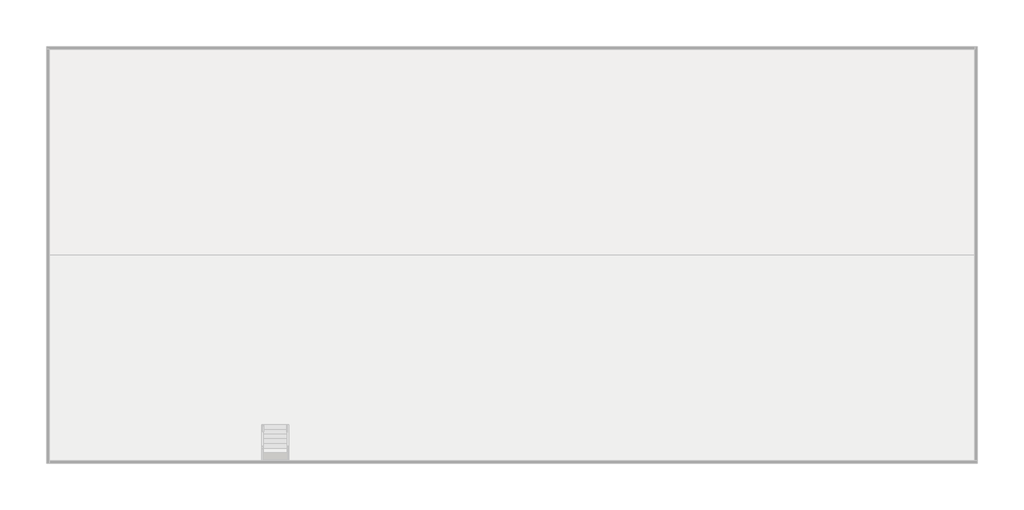
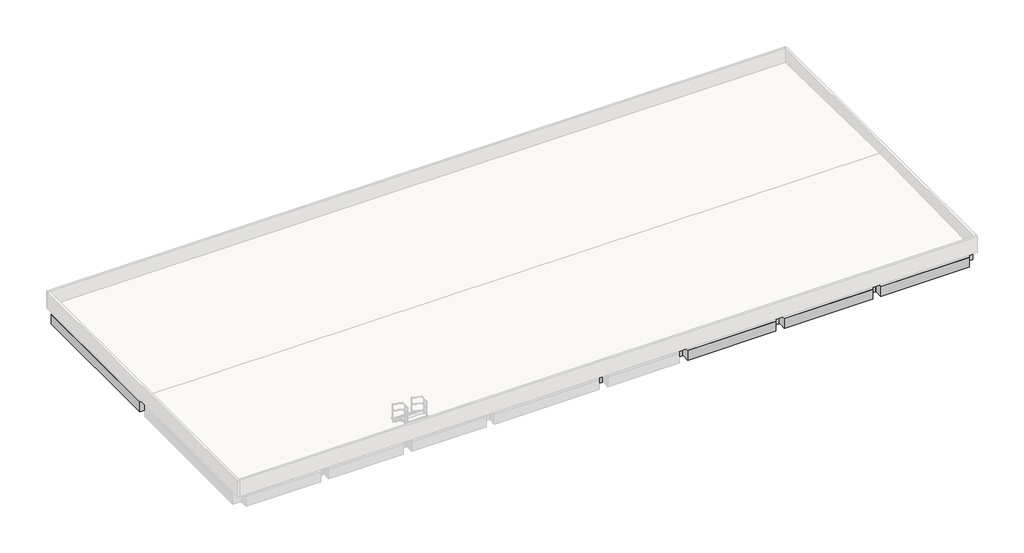
# One storey, part 2 of 3: 33 beams.
"""IFC4 building model written with IfcOpenShell, lengths in millimetres."""

import ifcopenshell
import ifcopenshell.guid

model = None  # the IFC model being written
_history = None  # IfcOwnerHistory: only IFC2X3 demands one
_inside = {}  # id of a spatial element -> (the spatial element, [elements in it])
_under = {}  # id of a project, library or spatial element -> (it, [spatial elements below it])
_declared = {}  # id of a project -> (the project, [libraries it declares])
_typed = {}  # id of a type object -> (the type object, [elements of that type])
_made_of = {}  # id of a material, layer set ... -> (it, [elements and type objects made of it])


def new_model(schema):
    """Start an empty IFC model of exactly this schema.

    Asked for "IFC4X3", IfcOpenShell would pick the latest addendum, in which some entities
    have other attributes; the version numbers below select the first issue.
    IFC2X3 requires an IfcOwnerHistory on every rooted entity: one is made here for all.
    """
    global model, _history
    if schema == "IFC4X3":
        model = ifcopenshell.file(schema_version=(4, 3, 0, 0))
    else:
        model = ifcopenshell.file(schema=schema)
    _inside.clear()
    _under.clear()
    _declared.clear()
    _typed.clear()
    _made_of.clear()
    _history = None
    if model.schema == "IFC2X3":
        org = make("IfcOrganization", Name="unknown")
        user = make(
            "IfcPersonAndOrganization",
            ThePerson=make("IfcPerson", FamilyName="unknown"),
            TheOrganization=org,
        )
        app = make(
            "IfcApplication",
            ApplicationDeveloper=org,
            Version="unknown",
            ApplicationFullName="unknown",
            ApplicationIdentifier="unknown",
        )
        _history = make(
            "IfcOwnerHistory",
            OwningUser=user,
            OwningApplication=app,
            ChangeAction="ADDED",
            CreationDate=0,
        )
    return model


def make(cls, **values):
    """One entity of the class cls with the attributes given. An attribute that is None is left unset."""
    return model.create_entity(
        cls, **{name: value for name, value in values.items() if value is not None}
    )


def rooted(cls, **values):
    """An entity with a GlobalId (a new one), such as an element, a storey or a relation."""
    return make(cls, GlobalId=ifcopenshell.guid.new(), OwnerHistory=_history, **values)


def si_unit(unit_type, name, prefix=None):
    """IfcSIUnit, for example si_unit("LENGTHUNIT", "METRE", prefix="MILLI")."""
    return make("IfcSIUnit", UnitType=unit_type, Prefix=prefix, Name=name)


def assignment(units):
    """IfcUnitAssignment: the units of a project."""
    return None if units is None else make("IfcUnitAssignment", Units=units)


def point(xyz):
    """IfcCartesianPoint."""
    return None if xyz is None else make("IfcCartesianPoint", Coordinates=xyz)


def direction(xyz):
    """IfcDirection."""
    return None if xyz is None else make("IfcDirection", DirectionRatios=xyz)


def frame(location, z_axis=None, x_axis=None):
    """IfcAxis2Placement3D, a coordinate frame: its origin and axes. An axis left out is left unset."""
    return make(
        "IfcAxis2Placement3D",
        Location=point(location),
        Axis=direction(z_axis),
        RefDirection=direction(x_axis),
    )


def origin():
    """The frame at (0, 0, 0) with its axes left unset."""
    return frame((0.0, 0.0, 0.0))


def place(relative_to, where):
    """IfcLocalPlacement: puts the frame where relative to a parent placement (None: the world)."""
    return make(
        "IfcLocalPlacement", PlacementRelTo=relative_to, RelativePlacement=where
    )


def context(
    kind, dimensions, precision=None, world=None, true_north=None, identifier=None
):
    """IfcGeometricRepresentationContext, for example the 3D "Model" context."""
    return make(
        "IfcGeometricRepresentationContext",
        ContextIdentifier=identifier,
        ContextType=kind,
        CoordinateSpaceDimension=dimensions,
        Precision=precision,
        WorldCoordinateSystem=world,
        TrueNorth=true_north,
    )


def project(units=None, contexts=None):
    """IfcProject with its units and contexts."""
    return rooted(
        "IfcProject",
        Name="project",
        RepresentationContexts=contexts,
        UnitsInContext=assignment(units),
    )


def spatial(cls, under=None, at=None, **own):
    """A site, building, storey or space (cls), placed at a placement, below another one or the project."""
    s = rooted(cls, ObjectPlacement=at, **own)
    if under is not None:
        _under.setdefault(under.id(), (under, []))[1].append(s)
    return s


def faces_of(points, faces, orient=None, outer=None):
    """IfcFace entities. A face is a list of loops; a loop is a list of indices into points, from 0.

    orient and outer hold one flag for each loop. By default every Orientation is true, the
    first loop of a face is its IfcFaceOuterBound and the others are IfcFaceBound.
    """
    made = []
    for i, loops in enumerate(faces):
        bounds = []
        for j, loop in enumerate(loops):
            is_outer = j == 0 if outer is None else outer[i][j]
            bounds.append(
                make(
                    "IfcFaceOuterBound" if is_outer else "IfcFaceBound",
                    Bound=make("IfcPolyLoop", Polygon=[points[k] for k in loop]),
                    Orientation=True if orient is None else orient[i][j],
                )
            )
        made.append(make("IfcFace", Bounds=bounds))
    return made


def faceted_brep(points, faces, orient=None, outer=None, voids=None):
    """IfcFacetedBrep: a solid bounded by flat faces; with voids (closed shells), ...WithVoids."""
    shared = [point(p) for p in points]
    hull = make("IfcClosedShell", CfsFaces=faces_of(shared, faces, orient, outer))
    if voids is None:
        return make("IfcFacetedBrep", Outer=hull)
    return make(
        "IfcFacetedBrepWithVoids",
        Outer=hull,
        Voids=[
            make(cls, CfsFaces=faces_of(shared, fs, o, b)) for cls, fs, o, b in voids
        ],
    )


def shape(context_of_items, identifier, shape_type, items):
    """IfcShapeRepresentation: the items that make up one representation, for example the "Body"."""
    return make(
        "IfcShapeRepresentation",
        ContextOfItems=context_of_items,
        RepresentationIdentifier=identifier,
        RepresentationType=shape_type,
        Items=items,
    )


def made_of(thing, what):
    """Note that an element or type object is made of a material, layer set ...; save() writes the relation."""
    if what is not None:
        _made_of.setdefault(what.id(), (what, []))[1].append(thing)
    return thing


def element(
    cls,
    number,
    at=None,
    inside=None,
    cuts=None,
    type_object=None,
    material=None,
    context=None,
    identifier="Body",
    shape_type=None,
    held_by="IfcProductDefinitionShape",
    body=None,
    shapes=None,
    **own,
):
    """One element of the class cls, such as IfcWall. Its Tag is "e" and its number.

    at: its placement. inside: the storey or other place that contains it. cuts: it is an
    opening in that element (IfcRelVoidsElement). A single representation is given by context,
    identifier, shape_type and body (its items); several are given by shapes. held_by: the class
    of the entity that holds the representations. save() writes the other relations.
    """
    e = rooted(cls, Tag="e%d" % number, ObjectPlacement=at, **own)
    if body is not None:
        shapes = [shape(context, identifier, shape_type, body)]
    if shapes is not None:
        e.Representation = make(held_by, Representations=shapes)
    if inside is not None:
        _inside.setdefault(inside.id(), (inside, []))[1].append(e)
    if cuts is not None:
        rooted(
            "IfcRelVoidsElement", RelatingBuildingElement=cuts, RelatedOpeningElement=e
        )
    if type_object is not None:
        _typed.setdefault(type_object.id(), (type_object, []))[1].append(e)
    return made_of(e, material)


def aggregate(whole, parts):
    """IfcRelAggregates: a whole, such as a stair, and the parts it consists of."""
    return rooted("IfcRelAggregates", RelatingObject=whole, RelatedObjects=parts)


def save(model, path):
    """Write the relations noted so far, then the file.

    IfcRelAggregates (storeys below a building ...), IfcRelContainedInSpatialStructure (elements
    in a storey), IfcRelDefinesByType, IfcRelAssociatesMaterial and IfcRelDeclares: one each for
    every whole, place, type object, material and project.
    """
    for whole, parts in _under.values():
        aggregate(whole, parts)
    for where, things in _inside.values():
        rooted(
            "IfcRelContainedInSpatialStructure",
            RelatedElements=things,
            RelatingStructure=where,
        )
    for kind, things in _typed.values():
        rooted("IfcRelDefinesByType", RelatedObjects=things, RelatingType=kind)
    for what, things in _made_of.values():
        rooted("IfcRelAssociatesMaterial", RelatedObjects=things, RelatingMaterial=what)
    for by, libraries in _declared.values():
        rooted("IfcRelDeclares", RelatingContext=by, RelatedDefinitions=libraries)
    model.write(path)


model = new_model("IFC4")

# Units and contexts
model_context = context("Model", 3, world=origin())
ifc_project = project(units=[si_unit("LENGTHUNIT", "METRE", prefix="MILLI")], contexts=[model_context])

# Site, building, storey
site = spatial("IfcSite", under=ifc_project)
building = spatial("IfcBuilding", under=site)
storey = spatial("IfcBuildingStorey", under=building, Name="TOC", Elevation=7649.9618634)

# Beams
placement = place(None, origin())
element("IfcBeam", 1, ObjectType="RC Beam_Rectangular : H_SB_AR_S16_B600xH900_RG9", at=placement, inside=storey, context=model_context, shape_type="Brep", body=[
    faceted_brep([(300.0, 24199.5208589, 6749.9618634), (300.0, 23749.5208589, 6749.9618634), (300.0, 23599.5208589, 6749.9618634), (300.0, 23599.5208589, 7499.9618634), (300.0, 24199.5208589, 7499.9618634), (5700.0, 23599.5208589, 6749.9618634), (5700.0, 23749.5208589, 6749.9618634), (5700.0, 24199.5208589, 6749.9618634), (5700.0, 24199.5208589, 7499.9618634), (5700.0, 23599.5208589, 7499.9618634), (2800.0, 23599.5208589, 7499.9618634), (3200.0, 23599.5208589, 7499.9618634), (2800.0, 23599.5208589, 6749.9618634), (3200.0, 23599.5208589, 6749.9618634)], [[[0, 1, 2, 3, 4]], [[5, 6, 7, 8, 9]], [[4, 3, 10, 11, 9, 8]], [[2, 12, 13, 5, 9, 11, 10, 3]], [[2, 1, 0, 7, 6, 5, 13, 12]], [[7, 0, 4, 8]]]),
])
element("IfcBeam", 2, ObjectType="RC Beam_Rectangular : H_SB_AR_S16_B600xH900_RG9", at=placement, inside=storey, context=model_context, shape_type="Brep", body=[
    faceted_brep([(6300.0, 24199.5208589, 6749.9618634), (6300.0, 23749.5208589, 6749.9618634), (6300.0, 23599.5208589, 6749.9618634), (6300.0, 23599.5208589, 7499.9618634), (6300.0, 24199.5208589, 7499.9618634), (11700.0, 23599.5208589, 6749.9618634), (11700.0, 23749.5208589, 6749.9618634), (11700.0, 24199.5208589, 6749.9618634), (11700.0, 24199.5208589, 7499.9618634), (11700.0, 23599.5208589, 7499.9618634), (8800.0, 23599.5208589, 7499.9618634), (9200.0, 23599.5208589, 7499.9618634), (8800.0, 23599.5208589, 6749.9618634), (9200.0, 23599.5208589, 6749.9618634)], [[[0, 1, 2, 3, 4]], [[5, 6, 7, 8, 9]], [[4, 3, 10, 11, 9, 8]], [[2, 12, 13, 5, 9, 11, 10, 3]], [[2, 1, 0, 7, 6, 5, 13, 12]], [[7, 0, 4, 8]]]),
])
element("IfcBeam", 3, ObjectType="RC Beam_Rectangular : H_SB_AR_S16_B600xH900_RG9", at=placement, inside=storey, context=model_context, shape_type="Brep", body=[
    faceted_brep([(12300.0, 24199.5208589, 6749.9618634), (12300.0, 23749.5208589, 6749.9618634), (12300.0, 23599.5208589, 6749.9618634), (12300.0, 23599.5208589, 7499.9618634), (12300.0, 24199.5208589, 7499.9618634), (17700.0, 23599.5208589, 6749.9618634), (17700.0, 23749.5208589, 6749.9618634), (17700.0, 24199.5208589, 6749.9618634), (17700.0, 24199.5208589, 7499.9618634), (17700.0, 23599.5208589, 7499.9618634), (14800.0, 23599.5208589, 7499.9618634), (15200.0, 23599.5208589, 7499.9618634), (14800.0, 23599.5208589, 6749.9618634), (15200.0, 23599.5208589, 6749.9618634)], [[[0, 1, 2, 3, 4]], [[5, 6, 7, 8, 9]], [[4, 3, 10, 11, 9, 8]], [[2, 12, 13, 5, 9, 11, 10, 3]], [[2, 1, 0, 7, 6, 5, 13, 12]], [[7, 0, 4, 8]]]),
])
element("IfcBeam", 4, ObjectType="RC Beam_Rectangular : H_SB_AR_S16_B600xH900_RG9", at=placement, inside=storey, context=model_context, shape_type="Brep", body=[
    faceted_brep([(18300.0, 24199.5208589, 6749.9618634), (18300.0, 23749.5208589, 6749.9618634), (18300.0, 23599.5208589, 6749.9618634), (18300.0, 23599.5208589, 7499.9618634), (18300.0, 24199.5208589, 7499.9618634), (25900.0, 23599.5208589, 6749.9618634), (25900.0, 23749.5208589, 6749.9618634), (25900.0, 24199.5208589, 6749.9618634), (25900.0, 24199.5208589, 7499.9618634), (25900.0, 23599.5208589, 7499.9618634), (21800.0, 23599.5208589, 7499.9618634), (22400.0, 23599.5208589, 7499.9618634), (21800.0, 23599.5208589, 6749.9618634), (22400.0, 23599.5208589, 6749.9618634)], [[[0, 1, 2, 3, 4]], [[5, 6, 7, 8, 9]], [[4, 3, 10, 11, 9, 8]], [[2, 12, 13, 5, 9, 11, 10, 3]], [[2, 1, 0, 7, 6, 5, 13, 12]], [[7, 0, 4, 8]]]),
])
element("IfcBeam", 5, ObjectType="RC Beam_Rectangular : H_SB_AR_S16_B600xH900_RG9", at=placement, inside=storey, context=model_context, shape_type="Brep", body=[
    faceted_brep([(26500.0, 24199.5208589, 6749.9618634), (26500.0, 23749.5208589, 6749.9618634), (26500.0, 23599.5208589, 6749.9618634), (26500.0, 23599.5208589, 7499.9618634), (26500.0, 24199.5208589, 7499.9618634), (31700.0, 23599.5208589, 6749.9618634), (31700.0, 23749.5208589, 6749.9618634), (31700.0, 24199.5208589, 6749.9618634), (31700.0, 24199.5208589, 7499.9618634), (31700.0, 23599.5208589, 7499.9618634), (28800.0, 23599.5208589, 7499.9618634), (29400.0, 23599.5208589, 7499.9618634), (28800.0, 23599.5208589, 6749.9618634), (29400.0, 23599.5208589, 6749.9618634)], [[[0, 1, 2, 3, 4]], [[5, 6, 7, 8, 9]], [[4, 3, 10, 11, 9, 8]], [[2, 12, 13, 5, 9, 11, 10, 3]], [[2, 1, 0, 7, 6, 5, 13, 12]], [[7, 0, 4, 8]]]),
])
element("IfcBeam", 6, ObjectType="RC Beam_Rectangular : H_SB_AR_S16_B600xH900_RG5", at=placement, inside=storey, context=model_context, shape_type="Brep", body=[
    faceted_brep([(26500.0, 8599.5208589, 6749.9618634), (26500.0, 8399.5208589, 6749.9618634), (26500.0, 7999.5208589, 6749.9618634), (26500.0, 7999.5208589, 7499.9618634), (26500.0, 8599.5208589, 7499.9618634), (31700.0, 7999.5208589, 6749.9618634), (31700.0, 8399.5208589, 6749.9618634), (31700.0, 8599.5208589, 6749.9618634), (31700.0, 8599.5208589, 7499.9618634), (31700.0, 7999.5208589, 7499.9618634), (28500.0, 7999.5208589, 7499.9618634), (28700.0, 7999.5208589, 7499.9618634), (28800.0, 7999.5208589, 7499.9618634), (29400.0, 7999.5208589, 7499.9618634), (29400.0, 8599.5208589, 7499.9618634), (28800.0, 8599.5208589, 7499.9618634), (28500.0, 7999.5208589, 6749.9618634), (28700.0, 7999.5208589, 6749.9618634), (28800.0, 7999.5208589, 6749.9618634), (29400.0, 7999.5208589, 6749.9618634), (28800.0, 8599.5208589, 6749.9618634), (29400.0, 8599.5208589, 6749.9618634)], [[[0, 1, 2, 3, 4]], [[5, 6, 7, 8, 9]], [[4, 3, 10, 11, 12, 13, 9, 8, 14, 15]], [[2, 16, 17, 18, 19, 5, 9, 13, 12, 11, 10, 3]], [[2, 1, 0, 20, 21, 7, 6, 5, 19, 18, 17, 16]], [[7, 21, 20, 0, 4, 15, 14, 8]]]),
])
element("IfcBeam", 7, ObjectType="RC Beam_Rectangular : H_SB_AR_S16_B600xH900_RG5", at=placement, inside=storey, context=model_context, shape_type="Brep", body=[
    faceted_brep([(32300.0, 8599.5208589, 6749.9618634), (32300.0, 8399.5208589, 6749.9618634), (32300.0, 7999.5208589, 6749.9618634), (32300.0, 7999.5208589, 7499.9618634), (32300.0, 8599.5208589, 7499.9618634), (38700.0, 7999.5208589, 6749.9618634), (38700.0, 8599.5208589, 6749.9618634), (38700.0, 8599.5208589, 7499.9618634), (38700.0, 7999.5208589, 7499.9618634), (35200.0, 7999.5208589, 7499.9618634), (35800.0, 7999.5208589, 7499.9618634), (36500.0, 7999.5208589, 7499.9618634), (36700.0, 7999.5208589, 7499.9618634), (36700.0, 8599.5208589, 7499.9618634), (36500.0, 8599.5208589, 7499.9618634), (35800.0, 8599.5208589, 7499.9618634), (35200.0, 8599.5208589, 7499.9618634), (33450.0, 8599.5208589, 7499.9618634), (33250.0, 8599.5208589, 7499.9618634), (35200.0, 7999.5208589, 6749.9618634), (35800.0, 7999.5208589, 6749.9618634), (36500.0, 7999.5208589, 6749.9618634), (36700.0, 7999.5208589, 6749.9618634), (35200.0, 8599.5208589, 6749.9618634), (35800.0, 8599.5208589, 6749.9618634), (36500.0, 8599.5208589, 6749.9618634), (36700.0, 8599.5208589, 6749.9618634)], [[[0, 1, 2, 3, 4]], [[5, 6, 7, 8]], [[4, 3, 9, 10, 11, 12, 8, 7, 13, 14, 15, 16, 17, 18]], [[2, 19, 20, 21, 22, 5, 8, 12, 11, 10, 9, 3]], [[2, 1, 0, 23, 24, 25, 26, 6, 5, 22, 21, 20, 19]], [[6, 26, 25, 24, 23, 0, 4, 18, 17, 16, 15, 14, 13, 7]]]),
])
element("IfcBeam", 8, ObjectType="RC Beam_Rectangular : H_SB_AR_S16_B600xH900_RG5", at=placement, inside=storey, context=model_context, shape_type="Brep", body=[
    faceted_brep([(39300.0, 8599.5208589, 6749.9618634), (39300.0, 8404.5208589, 6749.9618634), (39300.0, 8204.5208589, 6749.9618634), (39300.0, 7999.5208589, 6749.9618634), (39300.0, 7999.5208589, 7499.9618634), (39300.0, 8599.5208589, 7499.9618634), (45700.0, 7999.5208589, 6749.9618634), (45700.0, 8399.5208589, 6749.9618634), (45700.0, 8599.5208589, 6749.9618634), (45700.0, 8599.5208589, 7499.9618634), (45700.0, 7999.5208589, 7499.9618634), (41925.0, 7999.5208589, 7499.9618634), (42125.0, 7999.5208589, 7499.9618634), (42200.0, 7999.5208589, 7499.9618634), (42800.0, 7999.5208589, 7499.9618634), (43200.0, 7999.5208589, 7499.9618634), (43400.0, 7999.5208589, 7499.9618634), (42800.0, 8599.5208589, 7499.9618634), (42200.0, 8599.5208589, 7499.9618634), (41925.0, 7999.5208589, 6749.9618634), (42125.0, 7999.5208589, 6749.9618634), (42200.0, 7999.5208589, 6749.9618634), (42800.0, 7999.5208589, 6749.9618634), (43200.0, 7999.5208589, 6749.9618634), (43400.0, 7999.5208589, 6749.9618634), (42200.0, 8599.5208589, 6749.9618634), (42800.0, 8599.5208589, 6749.9618634), (45640.0, 8599.5208589, 6749.9618634)], [[[0, 1, 2, 3, 4, 5]], [[6, 7, 8, 9, 10]], [[5, 4, 11, 12, 13, 14, 15, 16, 10, 9, 17, 18]], [[3, 19, 20, 21, 22, 23, 24, 6, 10, 16, 15, 14, 13, 12, 11, 4]], [[3, 2, 1, 0, 25, 26, 27, 8, 7, 6, 24, 23, 22, 21, 20, 19]], [[8, 27, 26, 25, 0, 5, 18, 17, 9]]]),
])
element("IfcBeam", 9, ObjectType="RC Beam_Rectangular : H_SB_AR_S16_B600xH900_RG5", at=placement, inside=storey, context=model_context, shape_type="Brep", body=[
    faceted_brep([(46300.0, 8599.5208589, 6749.9618634), (46300.0, 8399.5208589, 6749.9618634), (46300.0, 7999.5208589, 6749.9618634), (46300.0, 7999.5208589, 7499.9618634), (46300.0, 8599.5208589, 7499.9618634), (52700.0, 7999.5208589, 6749.9618634), (52700.0, 8399.5208589, 6749.9618634), (52700.0, 8599.5208589, 6749.9618634), (52700.0, 8599.5208589, 7499.9618634), (52700.0, 7999.5208589, 7499.9618634), (49200.0, 7999.5208589, 7499.9618634), (49800.0, 7999.5208589, 7499.9618634), (52574.0, 7999.5208589, 7499.9618634), (52574.0, 8599.5208589, 7499.9618634), (50725.0, 8599.5208589, 7499.9618634), (50525.0, 8599.5208589, 7499.9618634), (49800.0, 8599.5208589, 7499.9618634), (49200.0, 8599.5208589, 7499.9618634), (49200.0, 7999.5208589, 6749.9618634), (49800.0, 7999.5208589, 6749.9618634), (52574.0, 7999.5208589, 6749.9618634), (49200.0, 8599.5208589, 6749.9618634), (49800.0, 8599.5208589, 6749.9618634)], [[[0, 1, 2, 3, 4]], [[5, 6, 7, 8, 9]], [[4, 3, 10, 11, 12, 9, 8, 13, 14, 15, 16, 17]], [[2, 18, 19, 20, 5, 9, 12, 11, 10, 3]], [[2, 1, 0, 21, 22, 7, 6, 5, 20, 19, 18]], [[7, 22, 21, 0, 4, 17, 16, 15, 14, 13, 8]]]),
])
element("IfcBeam", 10, ObjectType="RC Beam_Rectangular : H_SB_AR_S16_B600xH900_RG9", at=placement, inside=storey, context=model_context, shape_type="Brep", body=[
    faceted_brep([(32300.0, 799.5208589, 6749.9618634), (32300.0, 649.5208589, 6749.9618634), (32300.0, 199.5208589, 6749.9618634), (32300.0, 199.5208589, 7499.9618634), (32300.0, 799.5208589, 7499.9618634), (38700.0, 199.5208589, 6749.9618634), (38700.0, 649.5208589, 6749.9618634), (38700.0, 799.5208589, 6749.9618634), (38700.0, 799.5208589, 7499.9618634), (38700.0, 199.5208589, 7499.9618634), (36700.0, 799.5208589, 7499.9618634), (36500.0, 799.5208589, 7499.9618634), (35800.0, 799.5208589, 7499.9618634), (35200.0, 799.5208589, 7499.9618634), (35200.0, 799.5208589, 6749.9618634), (35800.0, 799.5208589, 6749.9618634)], [[[0, 1, 2, 3, 4]], [[5, 6, 7, 8, 9]], [[4, 3, 9, 8, 10, 11, 12, 13]], [[2, 5, 9, 3]], [[2, 1, 0, 14, 15, 7, 6, 5]], [[7, 15, 14, 0, 4, 13, 12, 11, 10, 8]]]),
])
element("IfcBeam", 11, ObjectType="RC Beam_Rectangular : H_SB_AR_S16_B600xH900_RG9", at=placement, inside=storey, context=model_context, shape_type="Brep", body=[
    faceted_brep([(39300.0, 799.5208589, 6749.9618634), (39300.0, 649.5208589, 6749.9618634), (39300.0, 199.5208589, 6749.9618634), (39300.0, 199.5208589, 7499.9618634), (39300.0, 799.5208589, 7499.9618634), (45700.0, 199.5208589, 6749.9618634), (45700.0, 649.5208589, 6749.9618634), (45700.0, 799.5208589, 6749.9618634), (45700.0, 799.5208589, 7499.9618634), (45700.0, 199.5208589, 7499.9618634), (43400.0, 799.5208589, 7499.9618634), (43200.0, 799.5208589, 7499.9618634), (42800.0, 799.5208589, 7499.9618634), (42200.0, 799.5208589, 7499.9618634), (42200.0, 799.5208589, 6749.9618634), (42800.0, 799.5208589, 6749.9618634)], [[[0, 1, 2, 3, 4]], [[5, 6, 7, 8, 9]], [[4, 3, 9, 8, 10, 11, 12, 13]], [[2, 5, 9, 3]], [[2, 1, 0, 14, 15, 7, 6, 5]], [[7, 15, 14, 0, 4, 13, 12, 11, 10, 8]]]),
])
element("IfcBeam", 12, ObjectType="RC Beam_Rectangular : H_SB_AR_S16_B600xH900_RG9", at=placement, inside=storey, context=model_context, shape_type="Brep", body=[
    faceted_brep([(46300.0, 799.5208589, 6749.9618634), (46300.0, 649.5208589, 6749.9618634), (46300.0, 199.5208589, 6749.9618634), (46300.0, 199.5208589, 7499.9618634), (46300.0, 799.5208589, 7499.9618634), (52700.0, 199.5208589, 6749.9618634), (52700.0, 649.5208589, 6749.9618634), (52700.0, 799.5208589, 6749.9618634), (52700.0, 799.5208589, 7499.9618634), (52700.0, 199.5208589, 7499.9618634), (49800.0, 799.5208589, 7499.9618634), (49200.0, 799.5208589, 7499.9618634), (46800.0, 799.5208589, 7499.9618634), (46600.0, 799.5208589, 7499.9618634), (49200.0, 799.5208589, 6749.9618634), (49800.0, 799.5208589, 6749.9618634)], [[[0, 1, 2, 3, 4]], [[5, 6, 7, 8, 9]], [[4, 3, 9, 8, 10, 11, 12, 13]], [[2, 5, 9, 3]], [[2, 1, 0, 14, 15, 7, 6, 5]], [[7, 15, 14, 0, 4, 13, 12, 11, 10, 8]]]),
])
element("IfcBeam", 13, ObjectType="RC Beam_Rectangular : H_SB_AR_S16_B600xH900_RG6", at=placement, inside=storey, context=model_context, shape_type="Brep", body=[
    faceted_brep([(-300.0, 12499.5208589, 6749.9618634), (150.0, 12499.5208589, 6749.9618634), (300.0, 12499.5208589, 6749.9618634), (300.0, 12499.5208589, 7499.9618634), (-300.0, 12499.5208589, 7499.9618634), (300.0, 23599.5208589, 6749.9618634), (150.0, 23599.5208589, 6749.9618634), (-300.0, 23599.5208589, 6749.9618634), (-300.0, 23599.5208589, 7499.9618634), (300.0, 23599.5208589, 7499.9618634), (300.0, 23473.5208589, 7499.9618634)], [[[0, 1, 2, 3, 4]], [[5, 6, 7, 8, 9]], [[4, 3, 10, 9, 8]], [[2, 5, 9, 10, 3]], [[2, 1, 0, 7, 6, 5]], [[7, 0, 4, 8]]]),
])
element("IfcBeam", 14, ObjectType="RC Beam_Rectangular : H_SB_AR_S16_B400xH900_RG1", at=placement, inside=storey, context=model_context, shape_type="Brep", body=[
    faceted_brep([(6200.0, 23599.5208589, 7499.9618634), (5800.0, 23599.5208589, 7499.9618634), (5800.0, 23473.5208589, 7499.9618634), (5800.0, 12499.5208589, 7499.9618634), (6200.0, 12499.5208589, 7499.9618634), (6200.0, 23473.5208589, 7499.9618634), (6200.0, 23599.5208589, 6749.9618634), (5800.0, 23599.5208589, 6749.9618634), (5800.0, 12499.5208589, 6749.9618634), (6200.0, 12499.5208589, 6749.9618634), (6200.0, 23473.5208589, 6749.9618634), (5800.0, 23473.5208589, 6749.9618634)], [[[0, 1, 2, 3, 4, 5]], [[6, 7, 1, 0]], [[8, 9, 4, 3]], [[9, 10, 6, 0, 5, 4]], [[8, 11, 7, 6, 10, 9]], [[7, 11, 8, 3, 2, 1]]]),
])
element("IfcBeam", 15, ObjectType="RC Beam_Rectangular : H_SB_AR_S16_B400xH900_RG1", at=placement, inside=storey, context=model_context, shape_type="Brep", body=[
    faceted_brep([(12200.0, 23599.5208589, 7499.9618634), (11800.0, 23599.5208589, 7499.9618634), (11800.0, 23473.5208589, 7499.9618634), (11800.0, 12499.5208589, 7499.9618634), (12200.0, 12499.5208589, 7499.9618634), (12200.0, 23473.5208589, 7499.9618634), (12200.0, 23599.5208589, 6749.9618634), (11800.0, 23599.5208589, 6749.9618634), (11800.0, 12499.5208589, 6749.9618634), (12200.0, 12499.5208589, 6749.9618634), (12200.0, 23473.5208589, 6749.9618634), (11800.0, 23473.5208589, 6749.9618634)], [[[0, 1, 2, 3, 4, 5]], [[6, 7, 1, 0]], [[8, 9, 4, 3]], [[9, 10, 6, 0, 5, 4]], [[9, 8, 11, 7, 6, 10]], [[7, 11, 8, 3, 2, 1]]]),
])
element("IfcBeam", 16, ObjectType="RC Beam_Rectangular : H_SB_AR_S16_B600xH900_RG1A", at=placement, inside=storey, context=model_context, shape_type="Brep", body=[
    faceted_brep([(17700.0, 12499.5208589, 6749.9618634), (18100.0, 12499.5208589, 6749.9618634), (18300.0, 12499.5208589, 6749.9618634), (18300.0, 12499.5208589, 7499.9618634), (17700.0, 12499.5208589, 7499.9618634), (18300.0, 23473.5208589, 7499.9618634), (18300.0, 23599.5208589, 7499.9618634), (17700.0, 23599.5208589, 7499.9618634), (17700.0, 23473.5208589, 7499.9618634), (18300.0, 23599.5208589, 6749.9618634), (18100.0, 23599.5208589, 6749.9618634), (17700.0, 23599.5208589, 6749.9618634), (17700.0, 23473.5208589, 6749.9618634)], [[[0, 1, 2, 3, 4]], [[4, 3, 5, 6, 7, 8]], [[9, 10, 11, 7, 6]], [[2, 9, 6, 5, 3]], [[0, 12, 11, 10, 9, 2, 1]], [[11, 12, 0, 4, 8, 7]]]),
])
element("IfcBeam", 17, ObjectType="RC Beam_Rectangular : H_SB_AR_S16_B500xH900_RG3", at=placement, inside=storey, context=model_context, shape_type="Brep", body=[
    faceted_brep([(26450.0, 7999.5208589, 6749.9618634), (26300.0, 7999.5208589, 6749.9618634), (26100.0, 7999.5208589, 6749.9618634), (25950.0, 7999.5208589, 6749.9618634), (25950.0, 7999.5208589, 7499.9618634), (26450.0, 7999.5208589, 7499.9618634), (25950.0, 925.5208589, 7499.9618634), (25950.0, 799.5208589, 7499.9618634), (26450.0, 799.5208589, 7499.9618634), (26450.0, 925.5208589, 7499.9618634), (26450.0, 2637.0208589, 7499.9618634), (26450.0, 2837.0208589, 7499.9618634), (25950.0, 799.5208589, 6749.9618634), (26100.0, 799.5208589, 6749.9618634), (26300.0, 799.5208589, 6749.9618634), (26450.0, 799.5208589, 6749.9618634), (26450.0, 925.5208589, 6749.9618634), (26450.0, 2637.0208589, 6749.9618634), (26450.0, 2837.0208589, 6749.9618634), (25950.0, 925.5208589, 6749.9618634)], [[[0, 1, 2, 3, 4, 5]], [[5, 4, 6, 7, 8, 9, 10, 11]], [[12, 13, 14, 15, 8, 7]], [[15, 16, 17, 18, 0, 5, 11, 10, 9, 8]], [[12, 19, 3, 2, 1, 0, 18, 17, 16, 15, 14, 13]], [[3, 19, 12, 7, 6, 4]]]),
])
element("IfcBeam", 18, ObjectType="RC Beam_Rectangular : H_SB_AR_S16_B500xH900_RG2", at=placement, inside=storey, context=model_context, shape_type="Brep", body=[
    faceted_brep([(26450.0, 23599.5208589, 7499.9618634), (25950.0, 23599.5208589, 7499.9618634), (25950.0, 23473.5208589, 7499.9618634), (25950.0, 8599.5208589, 7499.9618634), (26450.0, 8599.5208589, 7499.9618634), (26450.0, 23473.5208589, 7499.9618634), (26450.0, 23599.5208589, 6749.9618634), (25950.0, 23599.5208589, 6749.9618634), (25950.0, 8599.5208589, 6749.9618634), (26450.0, 8599.5208589, 6749.9618634), (26450.0, 23473.5208589, 6749.9618634), (25950.0, 23473.5208589, 6749.9618634)], [[[0, 1, 2, 3, 4, 5]], [[6, 7, 1, 0]], [[8, 9, 4, 3]], [[9, 10, 6, 0, 5, 4]], [[6, 10, 9, 8, 11, 7]], [[7, 11, 8, 3, 2, 1]]]),
])
element("IfcBeam", 19, ObjectType="RC Beam_Rectangular : H_SB_AR_S16_B500xH900_RG3", at=placement, inside=storey, context=model_context, shape_type="Brep", body=[
    faceted_brep([(31750.0, 799.5208589, 7499.9618634), (32250.0, 799.5208589, 7499.9618634), (32250.0, 925.5208589, 7499.9618634), (32250.0, 7999.5208589, 7499.9618634), (31750.0, 7999.5208589, 7499.9618634), (31750.0, 799.5208589, 6749.9618634), (31900.0, 799.5208589, 6749.9618634), (32250.0, 799.5208589, 6749.9618634), (32250.0, 7999.5208589, 6749.9618634), (31900.0, 7999.5208589, 6749.9618634), (31750.0, 7999.5208589, 6749.9618634), (32250.0, 925.5208589, 6749.9618634)], [[[0, 1, 2, 3, 4]], [[5, 6, 7, 1, 0]], [[8, 9, 10, 4, 3]], [[7, 11, 8, 3, 2, 1]], [[5, 10, 9, 8, 11, 7, 6]], [[10, 5, 0, 4]]]),
])
element("IfcBeam", 20, ObjectType="RC Beam_Rectangular : H_SB_AR_S16_B500xH900_RG2", at=placement, inside=storey, context=model_context, shape_type="Brep", body=[
    faceted_brep([(32250.0, 23599.5208589, 7499.9618634), (31750.0, 23599.5208589, 7499.9618634), (31750.0, 23473.5208589, 7499.9618634), (31750.0, 8599.5208589, 7499.9618634), (32250.0, 8599.5208589, 7499.9618634), (32250.0, 23473.5208589, 7499.9618634), (32250.0, 23599.5208589, 6749.9618634), (31750.0, 23599.5208589, 6749.9618634), (31750.0, 8599.5208589, 6749.9618634), (32250.0, 8599.5208589, 6749.9618634), (32250.0, 23473.5208589, 6749.9618634), (31750.0, 23473.5208589, 6749.9618634)], [[[0, 1, 2, 3, 4, 5]], [[6, 7, 1, 0]], [[8, 9, 4, 3]], [[9, 10, 6, 0, 5, 4]], [[8, 11, 7, 6, 10, 9]], [[7, 11, 8, 3, 2, 1]]]),
])
element("IfcBeam", 21, ObjectType="RC Beam_Rectangular : H_SB_AR_S16_B500xH900_RG3", at=placement, inside=storey, context=model_context, shape_type="Brep", body=[
    faceted_brep([(38750.0, 799.5208589, 7499.9618634), (39250.0, 799.5208589, 7499.9618634), (39250.0, 925.5208589, 7499.9618634), (39250.0, 4649.5208589, 7499.9618634), (39250.0, 4849.5208589, 7499.9618634), (39250.0, 7999.5208589, 7499.9618634), (38750.0, 7999.5208589, 7499.9618634), (38750.0, 3543.8249516, 7499.9618634), (38750.0, 3343.8249516, 7499.9618634), (38750.0, 925.5208589, 7499.9618634), (38750.0, 799.5208589, 6749.9618634), (38900.0, 799.5208589, 6749.9618634), (39100.0, 799.5208589, 6749.9618634), (39250.0, 799.5208589, 6749.9618634), (39250.0, 7999.5208589, 6749.9618634), (39100.0, 7999.5208589, 6749.9618634), (38900.0, 7999.5208589, 6749.9618634), (38750.0, 7999.5208589, 6749.9618634), (39250.0, 925.5208589, 6749.9618634), (39250.0, 4649.5208589, 6749.9618634), (39250.0, 4849.5208589, 6749.9618634), (38750.0, 925.5208589, 6749.9618634), (38750.0, 3343.8249516, 6749.9618634), (38750.0, 3543.8249516, 6749.9618634)], [[[0, 1, 2, 3, 4, 5, 6, 7, 8, 9]], [[10, 11, 12, 13, 1, 0]], [[14, 15, 16, 17, 6, 5]], [[13, 18, 19, 20, 14, 5, 4, 3, 2, 1]], [[10, 21, 22, 23, 17, 16, 15, 14, 20, 19, 18, 13, 12, 11]], [[17, 23, 22, 21, 10, 0, 9, 8, 7, 6]]]),
])
element("IfcBeam", 22, ObjectType="RC Beam_Rectangular : H_SB_AR_S16_B500xH900_RG3", at=placement, inside=storey, context=model_context, shape_type="Brep", body=[
    faceted_brep([(45750.0, 799.5208589, 7499.9618634), (46250.0, 799.5208589, 7499.9618634), (46250.0, 925.5208589, 7499.9618634), (46250.0, 4649.5208589, 7499.9618634), (46250.0, 4849.5208589, 7499.9618634), (46250.0, 6599.5208589, 7499.9618634), (46250.0, 6799.5208589, 7499.9618634), (46250.0, 7999.5208589, 7499.9618634), (45750.0, 7999.5208589, 7499.9618634), (45750.0, 6799.5208589, 7499.9618634), (45750.0, 6599.5208589, 7499.9618634), (45750.0, 4849.5208589, 7499.9618634), (45750.0, 4649.5208589, 7499.9618634), (45750.0, 925.5208589, 7499.9618634), (45750.0, 799.5208589, 6749.9618634), (46250.0, 799.5208589, 6749.9618634), (46250.0, 7999.5208589, 6749.9618634), (45750.0, 7999.5208589, 6749.9618634), (46250.0, 925.5208589, 6749.9618634), (46250.0, 4649.5208589, 6749.9618634), (46250.0, 4849.5208589, 6749.9618634), (46250.0, 6599.5208589, 6749.9618634), (46250.0, 6799.5208589, 6749.9618634), (45750.0, 925.5208589, 6749.9618634), (45750.0, 4649.5208589, 6749.9618634), (45750.0, 4849.5208589, 6749.9618634), (45750.0, 6599.5208589, 6749.9618634), (45750.0, 6799.5208589, 6749.9618634)], [[[0, 1, 2, 3, 4, 5, 6, 7, 8, 9, 10, 11, 12, 13]], [[14, 15, 1, 0]], [[16, 17, 8, 7]], [[15, 18, 19, 20, 21, 22, 16, 7, 6, 5, 4, 3, 2, 1]], [[14, 23, 24, 25, 26, 27, 17, 16, 22, 21, 20, 19, 18, 15]], [[17, 27, 26, 25, 24, 23, 14, 0, 13, 12, 11, 10, 9, 8]]]),
])
element("IfcBeam", 23, ObjectType="RC Beam_Rectangular : H_SB_AR_S16_B600xH900_RG8", at=placement, inside=storey, context=model_context, shape_type="Brep", body=[
    faceted_brep([(53300.0, 7999.5208589, 6749.9618634), (52850.0, 7999.5208589, 6749.9618634), (52700.0, 7999.5208589, 6749.9618634), (52700.0, 7999.5208589, 7499.9618634), (53300.0, 7999.5208589, 7499.9618634), (52700.0, 799.5208589, 6749.9618634), (52850.0, 799.5208589, 6749.9618634), (53300.0, 799.5208589, 6749.9618634), (53300.0, 799.5208589, 7499.9618634), (52700.0, 799.5208589, 7499.9618634), (52700.0, 925.5208589, 7499.9618634)], [[[0, 1, 2, 3, 4]], [[5, 6, 7, 8, 9]], [[4, 3, 10, 9, 8]], [[7, 0, 4, 8]], [[2, 1, 0, 7, 6, 5]], [[2, 5, 9, 10, 3]]]),
])
element("IfcBeam", 24, ObjectType="RC Beam_Rectangular : H_SB_AR_S16_B600xH900_RG5A", at=placement, inside=storey, context=model_context, shape_type="Brep", body=[
    faceted_brep([(18300.0, 7999.5208589, 6749.9618634), (21800.0, 7999.5208589, 6749.9618634), (22400.0, 7999.5208589, 6749.9618634), (25900.0, 7999.5208589, 6749.9618634), (25900.0, 7999.5208589, 7499.9618634), (22400.0, 7999.5208589, 7499.9618634), (21800.0, 7999.5208589, 7499.9618634), (18300.0, 7999.5208589, 7499.9618634), (25900.0, 8599.5208589, 6749.9618634), (25900.0, 8399.5208589, 6749.9618634), (18300.0, 8399.5208589, 6749.9618634), (18300.0, 8599.5208589, 6749.9618634), (21800.0, 8599.5208589, 6749.9618634), (22400.0, 8599.5208589, 6749.9618634), (18300.0, 8599.5208589, 7499.9618634), (21800.0, 8599.5208589, 7499.9618634), (22400.0, 8599.5208589, 7499.9618634), (25900.0, 8599.5208589, 7499.9618634)], [[[0, 1, 2, 3, 4, 5, 6, 7]], [[8, 9, 3, 2, 1, 0, 10, 11, 12, 13]], [[8, 13, 12, 11, 14, 15, 16, 17]], [[3, 9, 8, 17, 4]], [[7, 6, 5, 4, 17, 16, 15, 14]], [[11, 10, 0, 7, 14]]]),
])
element("IfcBeam", 25, ObjectType="RC Beam_Rectangular : H_SB_AR_S16_B400xH900_RB1", at=placement, inside=storey, context=model_context, shape_type="Brep", body=[
    faceted_brep([(2800.0, 23599.5208589, 6749.9618634), (2800.0, 23473.5208589, 6749.9618634), (2800.0, 12499.5208589, 6749.9618634), (2800.0, 12499.5208589, 7499.9618634), (2800.0, 23473.5208589, 7499.9618634), (2800.0, 23599.5208589, 7499.9618634), (3200.0, 12499.5208589, 6749.9618634), (3200.0, 23599.5208589, 6749.9618634), (3200.0, 23473.5208589, 6749.9618634), (3200.0, 23599.5208589, 7499.9618634), (3200.0, 23473.5208589, 7499.9618634), (3200.0, 12499.5208589, 7499.9618634)], [[[0, 1, 2, 3, 4, 5]], [[6, 2, 1, 0, 7, 8]], [[6, 8, 7, 9, 10, 11]], [[2, 6, 11, 3]], [[7, 0, 5, 9]], [[5, 4, 3, 11, 10, 9]]]),
])
element("IfcBeam", 26, ObjectType="RC Beam_Rectangular : H_SB_AR_S16_B400xH900_RB1", at=placement, inside=storey, context=model_context, shape_type="Brep", body=[
    faceted_brep([(8800.0, 23599.5208589, 6749.9618634), (8800.0, 23473.5208589, 6749.9618634), (8800.0, 12499.5208589, 6749.9618634), (8800.0, 12499.5208589, 7499.9618634), (8800.0, 23473.5208589, 7499.9618634), (8800.0, 23599.5208589, 7499.9618634), (9200.0, 12499.5208589, 6749.9618634), (9200.0, 23599.5208589, 6749.9618634), (9200.0, 23473.5208589, 6749.9618634), (9200.0, 23599.5208589, 7499.9618634), (9200.0, 23473.5208589, 7499.9618634), (9200.0, 12499.5208589, 7499.9618634)], [[[0, 1, 2, 3, 4, 5]], [[6, 2, 1, 0, 7, 8]], [[6, 8, 7, 9, 10, 11]], [[2, 6, 11, 3]], [[7, 0, 5, 9]], [[5, 4, 3, 11, 10, 9]]]),
])
element("IfcBeam", 27, ObjectType="RC Beam_Rectangular : H_SB_AR_S16_B400xH900_RB1", at=placement, inside=storey, context=model_context, shape_type="Brep", body=[
    faceted_brep([(14800.0, 23599.5208589, 6749.9618634), (14800.0, 23473.5208589, 6749.9618634), (14800.0, 12499.5208589, 6749.9618634), (14800.0, 12499.5208589, 7499.9618634), (14800.0, 23473.5208589, 7499.9618634), (14800.0, 23599.5208589, 7499.9618634), (15200.0, 12499.5208589, 6749.9618634), (15200.0, 23599.5208589, 6749.9618634), (15200.0, 23473.5208589, 6749.9618634), (15200.0, 23599.5208589, 7499.9618634), (15200.0, 23473.5208589, 7499.9618634), (15200.0, 12499.5208589, 7499.9618634)], [[[0, 1, 2, 3, 4, 5]], [[6, 2, 1, 0, 7, 8]], [[6, 8, 7, 9, 10, 11]], [[2, 6, 11, 3]], [[7, 0, 5, 9]], [[5, 4, 3, 11, 10, 9]]]),
])
element("IfcBeam", 28, ObjectType="RC Beam_Rectangular : H_SB_AR_S16_B600xH900_RB2", at=placement, inside=storey, context=model_context, shape_type="Brep", body=[
    faceted_brep([(21800.0, 23599.5208589, 6749.9618634), (21800.0, 23473.5208589, 6749.9618634), (21800.0, 8599.5208589, 6749.9618634), (21800.0, 8599.5208589, 7499.9618634), (21800.0, 23473.5208589, 7499.9618634), (21800.0, 23599.5208589, 7499.9618634), (22400.0, 8599.5208589, 6749.9618634), (22400.0, 23599.5208589, 6749.9618634), (22400.0, 23473.5208589, 6749.9618634), (22400.0, 23599.5208589, 7499.9618634), (22400.0, 23473.5208589, 7499.9618634), (22400.0, 8599.5208589, 7499.9618634)], [[[0, 1, 2, 3, 4, 5]], [[6, 2, 1, 0, 7, 8]], [[6, 8, 7, 9, 10, 11]], [[2, 6, 11, 3]], [[7, 0, 5, 9]], [[5, 4, 3, 11, 10, 9]]]),
])
element("IfcBeam", 29, ObjectType="RC Beam_Rectangular : H_SB_AR_S16_B600xH900_RB2", at=placement, inside=storey, context=model_context, shape_type="Brep", body=[
    faceted_brep([(28800.0, 23599.5208589, 6749.9618634), (28800.0, 23473.5208589, 6749.9618634), (28800.0, 8599.5208589, 6749.9618634), (28800.0, 8599.5208589, 7499.9618634), (28800.0, 23473.5208589, 7499.9618634), (28800.0, 23599.5208589, 7499.9618634), (29400.0, 8599.5208589, 6749.9618634), (29400.0, 23599.5208589, 6749.9618634), (29400.0, 23473.5208589, 6749.9618634), (29400.0, 23599.5208589, 7499.9618634), (29400.0, 23473.5208589, 7499.9618634), (29400.0, 8599.5208589, 7499.9618634)], [[[0, 1, 2, 3, 4, 5]], [[6, 2, 1, 0, 7, 8]], [[6, 8, 7, 9, 10, 11]], [[2, 6, 11, 3]], [[7, 0, 5, 9]], [[5, 4, 3, 11, 10, 9]]]),
])
element("IfcBeam", 30, ObjectType="RC Beam_Rectangular : H_SB_AR_S16_B600xH900_RB3", at=placement, inside=storey, context=model_context, shape_type="Brep", body=[
    faceted_brep([(28800.0, 7999.5208589, 6749.9618634), (28800.0, 4999.0208589, 6749.9618634), (28800.0, 4799.0208589, 6749.9618634), (28800.0, 925.5208589, 6749.9618634), (28800.0, 799.5208589, 6749.9618634), (28800.0, 799.5208589, 7499.9618634), (28800.0, 925.5208589, 7499.9618634), (28800.0, 4799.0208589, 7499.9618634), (28800.0, 4999.0208589, 7499.9618634), (28800.0, 7999.5208589, 7499.9618634), (29400.0, 7999.5208589, 6749.9618634), (29400.0, 4999.0208589, 6749.9618634), (29400.0, 4799.0208589, 6749.9618634), (29400.0, 925.5208589, 6749.9618634), (29400.0, 799.5208589, 6749.9618634), (29400.0, 7999.5208589, 7499.9618634), (29400.0, 4999.0208589, 7499.9618634), (29400.0, 4799.0208589, 7499.9618634), (29400.0, 925.5208589, 7499.9618634), (29400.0, 799.5208589, 7499.9618634)], [[[0, 1, 2, 3, 4, 5, 6, 7, 8, 9]], [[0, 10, 11, 12, 13, 14, 4, 3, 2, 1]], [[14, 13, 12, 11, 10, 15, 16, 17, 18, 19]], [[10, 0, 9, 15]], [[4, 14, 19, 5]], [[9, 8, 7, 6, 5, 19, 18, 17, 16, 15]]]),
])
element("IfcBeam", 31, ObjectType="RC Beam_Rectangular : H_SB_AR_S16_B600xH900_RB3", at=placement, inside=storey, context=model_context, shape_type="Brep", body=[
    faceted_brep([(35200.0, 7999.5208589, 6749.9618634), (35200.0, 925.5208589, 6749.9618634), (35200.0, 799.5208589, 6749.9618634), (35200.0, 799.5208589, 7499.9618634), (35200.0, 925.5208589, 7499.9618634), (35200.0, 7999.5208589, 7499.9618634), (35800.0, 7999.5208589, 6749.9618634), (35800.0, 925.5208589, 6749.9618634), (35800.0, 799.5208589, 6749.9618634), (35800.0, 7999.5208589, 7499.9618634), (35800.0, 925.5208589, 7499.9618634), (35800.0, 799.5208589, 7499.9618634)], [[[0, 1, 2, 3, 4, 5]], [[0, 6, 7, 8, 2, 1]], [[8, 7, 6, 9, 10, 11]], [[6, 0, 5, 9]], [[2, 8, 11, 3]], [[5, 4, 3, 11, 10, 9]]]),
])
element("IfcBeam", 32, ObjectType="RC Beam_Rectangular : H_SB_AR_S16_B600xH900_RB3", at=placement, inside=storey, context=model_context, shape_type="Brep", body=[
    faceted_brep([(42200.0, 7999.5208589, 6749.9618634), (42200.0, 6274.5208589, 6749.9618634), (42200.0, 6074.5208589, 6749.9618634), (42200.0, 4849.5208589, 6749.9618634), (42200.0, 4649.5208589, 6749.9618634), (42200.0, 925.5208589, 6749.9618634), (42200.0, 799.5208589, 6749.9618634), (42200.0, 799.5208589, 7499.9618634), (42200.0, 925.5208589, 7499.9618634), (42200.0, 4649.5208589, 7499.9618634), (42200.0, 4849.5208589, 7499.9618634), (42200.0, 6074.5208589, 7499.9618634), (42200.0, 6274.5208589, 7499.9618634), (42200.0, 7999.5208589, 7499.9618634), (42800.0, 7999.5208589, 6749.9618634), (42800.0, 6274.5208589, 6749.9618634), (42800.0, 6074.5208589, 6749.9618634), (42800.0, 4849.5208589, 6749.9618634), (42800.0, 4649.5208589, 6749.9618634), (42800.0, 925.5208589, 6749.9618634), (42800.0, 799.5208589, 6749.9618634), (42800.0, 7999.5208589, 7499.9618634), (42800.0, 6274.5208589, 7499.9618634), (42800.0, 6074.5208589, 7499.9618634), (42800.0, 4849.5208589, 7499.9618634), (42800.0, 4649.5208589, 7499.9618634), (42800.0, 925.5208589, 7499.9618634), (42800.0, 799.5208589, 7499.9618634)], [[[0, 1, 2, 3, 4, 5, 6, 7, 8, 9, 10, 11, 12, 13]], [[0, 14, 15, 16, 17, 18, 19, 20, 6, 5, 4, 3, 2, 1]], [[20, 19, 18, 17, 16, 15, 14, 21, 22, 23, 24, 25, 26, 27]], [[14, 0, 13, 21]], [[6, 20, 27, 7]], [[13, 12, 11, 10, 9, 8, 7, 27, 26, 25, 24, 23, 22, 21]]]),
])
element("IfcBeam", 33, ObjectType="RC Beam_Rectangular : H_SB_AR_S16_B600xH900_RB3", at=placement, inside=storey, context=model_context, shape_type="Brep", body=[
    faceted_brep([(49200.0, 7999.5208589, 6749.9618634), (49200.0, 925.5208589, 6749.9618634), (49200.0, 799.5208589, 6749.9618634), (49200.0, 799.5208589, 7499.9618634), (49200.0, 925.5208589, 7499.9618634), (49200.0, 7999.5208589, 7499.9618634), (49800.0, 7999.5208589, 6749.9618634), (49800.0, 925.5208589, 6749.9618634), (49800.0, 799.5208589, 6749.9618634), (49800.0, 7999.5208589, 7499.9618634), (49800.0, 925.5208589, 7499.9618634), (49800.0, 799.5208589, 7499.9618634)], [[[0, 1, 2, 3, 4, 5]], [[0, 6, 7, 8, 2, 1]], [[8, 7, 6, 9, 10, 11]], [[6, 0, 5, 9]], [[2, 8, 11, 3]], [[5, 4, 3, 11, 10, 9]]]),
])

save(model, "model.ifc")

# Revit data of these elements
# Type "RC Beam_Rectangular : H_SB_AR_S16_B600xH900_RG9"
#   중앙부 하부근 = ""
#   중앙부 상부근 = ""
#   중앙부 보조근 = ""
#   중앙부 늑근 = ""
#   외단부 하부근 = ""
#   외단부 상부근 = ""
#   외단부 보조근 = ""
#   외단부 늑근 = ""
#   부호 = "TG3"
#   내단부 하부근 = ""
#   내단부 상부근 = ""
#   내단부 보조근 = ""
#   내단부 늑근 = ""
#   ALL 하부근 = "3-D20"
#   ALL 상부근 = "3-D20"
#   ALL 보조근 = ""
#   ALL 늑근 = "2-D10 @120"
#   Width = 600 mm
#   Height = 900 mm
#   Length [instance default] = 1524 mm
#   b = 600 mm
#   h = 900 mm
#   hec_material3 [instance default] = none
#   hec_material2 [instance default] = none
#   hec_material1 [instance default] = none
#   Structural Material [instance default] = none
#   Assembly Code = ""
# Type "RC Beam_Rectangular : H_SB_AR_S16_B600xH900_RG5"
#   중앙부 하부근 = ""
#   중앙부 상부근 = ""
#   중앙부 보조근 = ""
#   중앙부 늑근 = ""
#   외단부 하부근 = ""
#   외단부 상부근 = ""
#   외단부 보조근 = ""
#   외단부 늑근 = ""
#   부호 = "TG3"
#   내단부 하부근 = ""
#   내단부 상부근 = ""
#   내단부 보조근 = ""
#   내단부 늑근 = ""
#   ALL 하부근 = "3-D20"
#   ALL 상부근 = "3-D20"
#   ALL 보조근 = ""
#   ALL 늑근 = "2-D10 @120"
#   Width = 600 mm
#   Height = 900 mm
#   Length [instance default] = 1524 mm
#   b = 600 mm
#   h = 900 mm
#   hec_material3 [instance default] = none
#   hec_material2 [instance default] = none
#   hec_material1 [instance default] = none
#   Structural Material [instance default] = none
#   Assembly Code = ""
# Type "RC Beam_Rectangular : H_SB_AR_S16_B600xH900_RG6"
#   중앙부 하부근 = ""
#   중앙부 상부근 = ""
#   중앙부 보조근 = ""
#   중앙부 늑근 = ""
#   외단부 하부근 = ""
#   외단부 상부근 = ""
#   외단부 보조근 = ""
#   외단부 늑근 = ""
#   부호 = "TG3"
#   내단부 하부근 = ""
#   내단부 상부근 = ""
#   내단부 보조근 = ""
#   내단부 늑근 = ""
#   ALL 하부근 = "3-D20"
#   ALL 상부근 = "3-D20"
#   ALL 보조근 = ""
#   ALL 늑근 = "2-D10 @120"
#   Width = 600 mm
#   Height = 900 mm
#   Length [instance default] = 1524 mm
#   b = 600 mm
#   h = 900 mm
#   hec_material3 [instance default] = none
#   hec_material2 [instance default] = none
#   hec_material1 [instance default] = none
#   Structural Material [instance default] = none
#   Assembly Code = ""
# Type "RC Beam_Rectangular : H_SB_AR_S16_B400xH900_RG1"
#   중앙부 하부근 = ""
#   중앙부 상부근 = ""
#   중앙부 보조근 = ""
#   중앙부 늑근 = ""
#   외단부 하부근 = ""
#   외단부 상부근 = ""
#   외단부 보조근 = ""
#   외단부 늑근 = ""
#   부호 = "TG3"
#   내단부 하부근 = ""
#   내단부 상부근 = ""
#   내단부 보조근 = ""
#   내단부 늑근 = ""
#   ALL 하부근 = "3-D20"
#   ALL 상부근 = "3-D20"
#   ALL 보조근 = ""
#   ALL 늑근 = "2-D10 @120"
#   Width = 400 mm
#   Height = 900 mm
#   Length [instance default] = 1524 mm
#   b = 400 mm
#   h = 900 mm
#   hec_material3 [instance default] = none
#   hec_material2 [instance default] = none
#   hec_material1 [instance default] = none
#   Structural Material [instance default] = none
#   Assembly Code = ""
# Type "RC Beam_Rectangular : H_SB_AR_S16_B600xH900_RG1A"
#   중앙부 하부근 = ""
#   중앙부 상부근 = ""
#   중앙부 보조근 = ""
#   중앙부 늑근 = ""
#   외단부 하부근 = ""
#   외단부 상부근 = ""
#   외단부 보조근 = ""
#   외단부 늑근 = ""
#   부호 = "TG3"
#   내단부 하부근 = ""
#   내단부 상부근 = ""
#   내단부 보조근 = ""
#   내단부 늑근 = ""
#   ALL 하부근 = "3-D20"
#   ALL 상부근 = "3-D20"
#   ALL 보조근 = ""
#   ALL 늑근 = "2-D10 @120"
#   Width = 600 mm
#   Height = 900 mm
#   Length [instance default] = 1524 mm
#   b = 600 mm
#   h = 900 mm
#   hec_material3 [instance default] = none
#   hec_material2 [instance default] = none
#   hec_material1 [instance default] = none
#   Structural Material [instance default] = none
#   Assembly Code = ""
# Type "RC Beam_Rectangular : H_SB_AR_S16_B500xH900_RG3"
#   중앙부 하부근 = ""
#   중앙부 상부근 = ""
#   중앙부 보조근 = ""
#   중앙부 늑근 = ""
#   외단부 하부근 = ""
#   외단부 상부근 = ""
#   외단부 보조근 = ""
#   외단부 늑근 = ""
#   부호 = "TG3"
#   내단부 하부근 = ""
#   내단부 상부근 = ""
#   내단부 보조근 = ""
#   내단부 늑근 = ""
#   ALL 하부근 = "3-D20"
#   ALL 상부근 = "3-D20"
#   ALL 보조근 = ""
#   ALL 늑근 = "2-D10 @120"
#   Width = 500 mm
#   Height = 900 mm
#   Length [instance default] = 1524 mm
#   b = 500 mm
#   h = 900 mm
#   hec_material3 [instance default] = none
#   hec_material2 [instance default] = none
#   hec_material1 [instance default] = none
#   Structural Material [instance default] = none
#   Assembly Code = ""
# Type "RC Beam_Rectangular : H_SB_AR_S16_B500xH900_RG2"
#   중앙부 하부근 = ""
#   중앙부 상부근 = ""
#   중앙부 보조근 = ""
#   중앙부 늑근 = ""
#   외단부 하부근 = ""
#   외단부 상부근 = ""
#   외단부 보조근 = ""
#   외단부 늑근 = ""
#   부호 = "TG3"
#   내단부 하부근 = ""
#   내단부 상부근 = ""
#   내단부 보조근 = ""
#   내단부 늑근 = ""
#   ALL 하부근 = "3-D20"
#   ALL 상부근 = "3-D20"
#   ALL 보조근 = ""
#   ALL 늑근 = "2-D10 @120"
#   Width = 500 mm
#   Height = 900 mm
#   Length [instance default] = 1524 mm
#   b = 500 mm
#   h = 900 mm
#   hec_material3 [instance default] = none
#   hec_material2 [instance default] = none
#   hec_material1 [instance default] = none
#   Structural Material [instance default] = none
#   Assembly Code = ""
# Type "RC Beam_Rectangular : H_SB_AR_S16_B600xH900_RG8"
#   중앙부 하부근 = ""
#   중앙부 상부근 = ""
#   중앙부 보조근 = ""
#   중앙부 늑근 = ""
#   외단부 하부근 = ""
#   외단부 상부근 = ""
#   외단부 보조근 = ""
#   외단부 늑근 = ""
#   부호 = "TG3"
#   내단부 하부근 = ""
#   내단부 상부근 = ""
#   내단부 보조근 = ""
#   내단부 늑근 = ""
#   ALL 하부근 = "3-D20"
#   ALL 상부근 = "3-D20"
#   ALL 보조근 = ""
#   ALL 늑근 = "2-D10 @120"
#   Width = 600 mm
#   Height = 900 mm
#   Length [instance default] = 1524 mm
#   b = 600 mm
#   h = 900 mm
#   hec_material3 [instance default] = none
#   hec_material2 [instance default] = none
#   hec_material1 [instance default] = none
#   Structural Material [instance default] = none
#   Assembly Code = ""
# Type "RC Beam_Rectangular : H_SB_AR_S16_B600xH900_RG5A"
#   중앙부 하부근 = ""
#   중앙부 상부근 = ""
#   중앙부 보조근 = ""
#   중앙부 늑근 = ""
#   외단부 하부근 = ""
#   외단부 상부근 = ""
#   외단부 보조근 = ""
#   외단부 늑근 = ""
#   부호 = "TG3"
#   내단부 하부근 = ""
#   내단부 상부근 = ""
#   내단부 보조근 = ""
#   내단부 늑근 = ""
#   ALL 하부근 = "3-D20"
#   ALL 상부근 = "3-D20"
#   ALL 보조근 = ""
#   ALL 늑근 = "2-D10 @120"
#   Width = 600 mm
#   Height = 900 mm
#   Length [instance default] = 1524 mm
#   b = 600 mm
#   h = 900 mm
#   hec_material3 [instance default] = none
#   hec_material2 [instance default] = none
#   hec_material1 [instance default] = none
#   Structural Material [instance default] = none
#   Assembly Code = ""
# Type "RC Beam_Rectangular : H_SB_AR_S16_B400xH900_RB1"
#   중앙부 하부근 = ""
#   중앙부 상부근 = ""
#   중앙부 보조근 = ""
#   중앙부 늑근 = ""
#   외단부 하부근 = ""
#   외단부 상부근 = ""
#   외단부 보조근 = ""
#   외단부 늑근 = ""
#   부호 = "TG3"
#   내단부 하부근 = ""
#   내단부 상부근 = ""
#   내단부 보조근 = ""
#   내단부 늑근 = ""
#   ALL 하부근 = "3-D20"
#   ALL 상부근 = "3-D20"
#   ALL 보조근 = ""
#   ALL 늑근 = "2-D10 @120"
#   Width = 400 mm
#   Height = 900 mm
#   Length [instance default] = 1524 mm
#   b = 400 mm
#   h = 900 mm
#   hec_material3 [instance default] = none
#   hec_material2 [instance default] = none
#   hec_material1 [instance default] = none
#   Structural Material [instance default] = none
#   Assembly Code = ""
# Type "RC Beam_Rectangular : H_SB_AR_S16_B600xH900_RB2"
#   중앙부 하부근 = ""
#   중앙부 상부근 = ""
#   중앙부 보조근 = ""
#   중앙부 늑근 = ""
#   외단부 하부근 = ""
#   외단부 상부근 = ""
#   외단부 보조근 = ""
#   외단부 늑근 = ""
#   부호 = "TG3"
#   내단부 하부근 = ""
#   내단부 상부근 = ""
#   내단부 보조근 = ""
#   내단부 늑근 = ""
#   ALL 하부근 = "3-D20"
#   ALL 상부근 = "3-D20"
#   ALL 보조근 = ""
#   ALL 늑근 = "2-D10 @120"
#   Width = 600 mm
#   Height = 900 mm
#   Length [instance default] = 1524 mm
#   b = 600 mm
#   h = 900 mm
#   hec_material3 [instance default] = none
#   hec_material2 [instance default] = none
#   hec_material1 [instance default] = none
#   Structural Material [instance default] = none
#   Assembly Code = ""
# Type "RC Beam_Rectangular : H_SB_AR_S16_B600xH900_RB3"
#   중앙부 하부근 = ""
#   중앙부 상부근 = ""
#   중앙부 보조근 = ""
#   중앙부 늑근 = ""
#   외단부 하부근 = ""
#   외단부 상부근 = ""
#   외단부 보조근 = ""
#   외단부 늑근 = ""
#   부호 = "TG3"
#   내단부 하부근 = ""
#   내단부 상부근 = ""
#   내단부 보조근 = ""
#   내단부 늑근 = ""
#   ALL 하부근 = "3-D20"
#   ALL 상부근 = "3-D20"
#   ALL 보조근 = ""
#   ALL 늑근 = "2-D10 @120"
#   Width = 600 mm
#   Height = 900 mm
#   Length [instance default] = 1524 mm
#   b = 600 mm
#   h = 900 mm
#   hec_material3 [instance default] = none
#   hec_material2 [instance default] = none
#   hec_material1 [instance default] = none
#   Structural Material [instance default] = none
#   Assembly Code = ""
# Elements 1, 2, 3, 4, 5, 10, 11, 12 (IfcBeam, "RC Beam_Rectangular : H_SB_AR_S16_B600xH900_RG9")
#   Comments = ""
#   hec_material3 = none
#   hec_material2 = none
#   hec_material1 = none
#   Structural Material = Concrete - Cast-in-Place Concrete - 35 MPa
#   Phase Created = New Construction
#   Materials on its faces: "Concrete - Cast-in-Place Concrete - 35 MPa"
# Elements 6, 7, 8, 9 (IfcBeam, "RC Beam_Rectangular : H_SB_AR_S16_B600xH900_RG5")
#   Comments = ""
#   hec_material3 = none
#   hec_material2 = none
#   hec_material1 = none
#   Structural Material = Concrete - Cast-in-Place Concrete - 35 MPa
#   Phase Created = New Construction
#   Materials on its faces: "Concrete - Cast-in-Place Concrete - 35 MPa"
# Element 13 (IfcBeam, "RC Beam_Rectangular : H_SB_AR_S16_B600xH900_RG6")
#   Comments = ""
#   hec_material3 = none
#   hec_material2 = none
#   hec_material1 = none
#   Structural Material = Concrete - Cast-in-Place Concrete - 35 MPa
#   Phase Created = New Construction
#   Materials on its faces: "Concrete - Cast-in-Place Concrete - 35 MPa"
# Elements 14, 15 (IfcBeam, "RC Beam_Rectangular : H_SB_AR_S16_B400xH900_RG1")
#   Comments = ""
#   hec_material3 = none
#   hec_material2 = none
#   hec_material1 = none
#   Structural Material = Concrete - Cast-in-Place Concrete - 35 MPa
#   Phase Created = New Construction
#   Materials on its faces: "Concrete - Cast-in-Place Concrete - 35 MPa"
# Element 16 (IfcBeam, "RC Beam_Rectangular : H_SB_AR_S16_B600xH900_RG1A")
#   Comments = ""
#   hec_material3 = none
#   hec_material2 = none
#   hec_material1 = none
#   Structural Material = Concrete - Cast-in-Place Concrete - 35 MPa
#   Phase Created = New Construction
#   Materials on its faces: "Concrete - Cast-in-Place Concrete - 35 MPa"
# Elements 17, 19, 21, 22 (IfcBeam, "RC Beam_Rectangular : H_SB_AR_S16_B500xH900_RG3")
#   Comments = ""
#   hec_material3 = none
#   hec_material2 = none
#   hec_material1 = none
#   Structural Material = Concrete - Cast-in-Place Concrete - 35 MPa
#   Phase Created = New Construction
#   Materials on its faces: "Concrete - Cast-in-Place Concrete - 35 MPa"
# Elements 18, 20 (IfcBeam, "RC Beam_Rectangular : H_SB_AR_S16_B500xH900_RG2")
#   Comments = ""
#   hec_material3 = none
#   hec_material2 = none
#   hec_material1 = none
#   Structural Material = Concrete - Cast-in-Place Concrete - 35 MPa
#   Phase Created = New Construction
#   Materials on its faces: "Concrete - Cast-in-Place Concrete - 35 MPa"
# Element 23 (IfcBeam, "RC Beam_Rectangular : H_SB_AR_S16_B600xH900_RG8")
#   Comments = ""
#   hec_material3 = none
#   hec_material2 = none
#   hec_material1 = none
#   Structural Material = Concrete - Cast-in-Place Concrete - 35 MPa
#   Phase Created = New Construction
#   Materials on its faces: "Concrete - Cast-in-Place Concrete - 35 MPa"
# Element 24 (IfcBeam, "RC Beam_Rectangular : H_SB_AR_S16_B600xH900_RG5A")
#   hec_material3 = none
#   hec_material2 = none
#   hec_material1 = none
#   Structural Material = Concrete - Cast-in-Place Concrete - 35 MPa
#   Phase Created = New Construction
#   Materials on its faces: "Concrete - Cast-in-Place Concrete - 35 MPa"
# Elements 25, 26, 27 (IfcBeam, "RC Beam_Rectangular : H_SB_AR_S16_B400xH900_RB1")
#   hec_material3 = none
#   hec_material2 = none
#   hec_material1 = none
#   Structural Material = Concrete - Cast-in-Place Concrete - 35 MPa
#   Phase Created = New Construction
#   Materials on its faces: "Concrete - Cast-in-Place Concrete - 35 MPa"
# Elements 28, 29 (IfcBeam, "RC Beam_Rectangular : H_SB_AR_S16_B600xH900_RB2")
#   hec_material3 = none
#   hec_material2 = none
#   hec_material1 = none
#   Structural Material = Concrete - Cast-in-Place Concrete - 35 MPa
#   Phase Created = New Construction
#   Materials on its faces: "Concrete - Cast-in-Place Concrete - 35 MPa"
# Elements 30, 31, 32, 33 (IfcBeam, "RC Beam_Rectangular : H_SB_AR_S16_B600xH900_RB3")
#   hec_material3 = none
#   hec_material2 = none
#   hec_material1 = none
#   Structural Material = Concrete - Cast-in-Place Concrete - 35 MPa
#   Phase Created = New Construction
#   Materials on its faces: "Concrete - Cast-in-Place Concrete - 35 MPa"
# Materials
#   "Concrete - Cast-in-Place Concrete - 35 MPa": class "Concrete", colour RGB 192 192 192, transparency 0, Cost = 0
